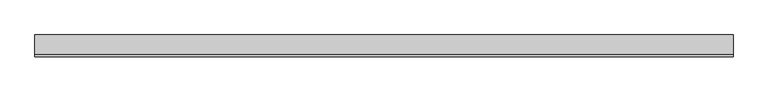
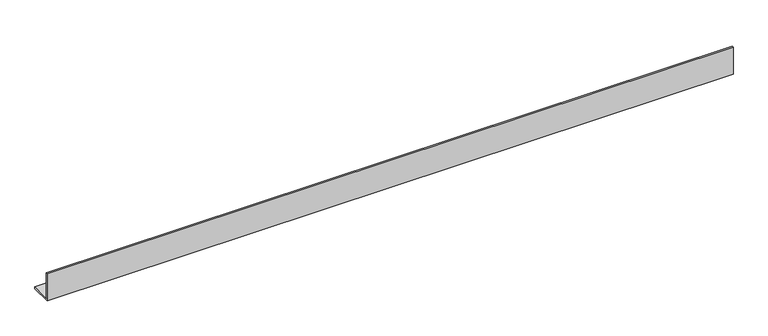
"""IFC4 building model written with IfcOpenShell, lengths in millimetres: proxy geometry, Generic Models 3:Generic Models 1:6:Generic Models 1:6 : Generic Models 3:Generic Models 1:300625:350611:Generic Models 1:6:Generic Models 1:6 : Generic Models 3:Generic Models 1:300625:350611 : Generic Models 3:Generic Models 1:6:Generic Models 1:6 : Generic Models 3:Generic Models 1:300625:350611:2 : Generic Models 3:Generic Models 1:6:Generic Models 1:6 : Generic Models 3:Generic Models 1:300625:350611:Generic Models 1:6:Generic Models 1:6 : Generic Models 3:Generic Models 1:300625:350611 : Generic Models 3:Generic Models 1:6:Generic Models 1:6 : Generic Models 3:Generic Models 1:300625:350611:301824."""

from ifc_helpers import new_model, si_unit, frame, origin, place, context, project, spatial, polyline, outline, extrude, source, transform, mapped, element, save


def generic_models_5076a2cb(model_context):
    return source(origin(), model_context, "Body", "SweptSolid", [
        extrude(outline(polyline([(-579000.6913841, 0.0), (-579000.6913841, 101.6), (-578994.3413841, 101.6), (-578994.3413841, 6.35), (-578924.4913841, 6.35), (-578924.4913841, 0.0), (-579000.6913841, 0.0)])), frame((593738.0867239, 0.0, 0.0), z_axis=(1.0, 0.0, 0.0), x_axis=(0.0, 1.0, 0.0)), (0.0, 0.0, 1.0), 2438.4),
    ])


if __name__ == "__main__":
    model = new_model("IFC4")
    model_context = context("Model", 3, world=origin())
    ifc_project = project(units=[si_unit("LENGTHUNIT", "METRE", prefix="MILLI")], contexts=[model_context])
    site = spatial("IfcSite", under=ifc_project)
    building = spatial("IfcBuilding", under=site)
    placement = place(None, origin())
    generic_models_shape = generic_models_5076a2cb(model_context)
    element("IfcBuildingElementProxy", 1, Name="Generic Models 3:Generic Models 1:6:Generic Models 1:6 : Generic Models 3:Generic Models 1:300625:350611:Generic Models 1:6:Generic Models 1:6 : Generic Models 3:Generic Models 1:300625:350611 : Generic Models 3:Generic Models 1:6:Generic Models 1:6 : Generic Models 3:Generic Models 1:300625:350611:2 : Generic Models 3:Generic Models 1:6:Generic Models 1:6 : Generic Models 3:Generic Models 1:300625:350611:Generic Models 1:6:Generic Models 1:6 : Generic Models 3:Generic Models 1:300625:350611 : Generic Models 3:Generic Models 1:6:Generic Models 1:6 : Generic Models 3:Generic Models 1:300625:350611:301824", ObjectType="Generic Models 3:Generic Models 1:6:Generic Models 1:6 : Generic Models 3:Generic Models 1:300625:350611:Generic Models 1:6:Generic Models 1:6 : Generic Models 3:Generic Models 1:300625:350611 : Generic Models 3:Generic Models 1:6:Generic Models 1:6 : Generic Models 3:Generic Models 1:300625:350611:2 : Generic Models 3:Generic Models 1:6:Generic Models 1:6 : Generic Models 3:Generic Models 1:300625:350611:Generic Models 1:6:Generic Models 1:6 : Generic Models 3:Generic Models 1:300625:350611 : Generic Models 3:Generic Models 1:6:Generic Models 1:6 : Generic Models 3:Generic Models 1:300625:350611:301824", at=placement, inside=building, context=model_context, shape_type="MappedRepresentation", body=[
        mapped(generic_models_shape, transform((0.0, 0.0, 0.0), x_axis=(1.0, 0.0, 0.0), y_axis=(0.0, 1.0, 0.0), z_axis=(0.0, 0.0, 1.0))),
    ])
    save(model, "model.ifc")

# Revit data of these elements
# Type "Generic Models 3:Generic Models 1:6:Generic Models 1:6 : Generic Models 3:Generic Models 1:300625:350611:Generic Models 1:6:Generic Models 1:6 : Generic Models 3:Generic Models 1:300625:350611 : Generic Models 3:Generic Models 1:6:Generic Models 1:6 : Generic Models 3:Generic Models 1:300625:350611:2 : Generic Models 3:Generic Models 1:6:Generic Models 1:6 : Generic Models 3:Generic Models 1:300625:350611:Generic Models 1:6:Generic Models 1:6 : Generic Models 3:Generic Models 1:300625:350611 : Generic Models 3:Generic Models 1:6:Generic Models 1:6 : Generic Models 3:Generic Models 1:300625:350611:301824"
#   NameOverride = "Generic Models 3:Generic Models 1:6:Generic Models 1:6 : Generic Models 3:Generic Models 1:300625:350611:Generic Models 1:6:Generic Models 1:6 : Generic Models 3:Generic Models 1:300625:350611 : Generic Models 3:Generic Models 1:6:Generic Models 1:6 : Generic Models 3:Generic Models 1:300625:350611:301824"
#   ObjectTypeOverride = "Generic Models 1:6:Generic Models 1:6 : Generic Models 3:Generic Models 1:300625:350611 : Generic Models 3:Generic Models 1:6:Generic Models 1:6 : Generic Models 3:Generic Models 1:300625:350611"
#   Reference = "Generic Models 1"
#   Tag = "301824"
# Element 1 (IfcBuildingElementProxy, "Generic Models 3:Generic Models 1:6:Generic Models 1:6 : Generic Models 3:Generic Models 1:300625:350611:Generic Models 1:6:Generic Models 1:6 : Generic Models 3:Generic Models 1:300625:350611 : Generic Models 3:Generic Models 1:6:Generic Models 1:6 : Generic Models 3:Generic Models 1:300625:350611:2 : Generic Models 3:Generic Models 1:6:Generic Models 1:6 : Generic Models 3:Generic Models 1:300625:350611:Generic Models 1:6:Generic Models 1:6 : Generic Models 3:Generic Models 1:300625:350611 : Generic Models 3:Generic Models 1:6:Generic Models 1:6 : Generic Models 3:Generic Models 1:300625:350611:301824")
#   Materials on its faces: "6\" Metal Stud Track_1"
# Materials
#   "6\" Metal Stud Track_1": class "Unassigned", colour RGB 120 120 120, transparency 0
